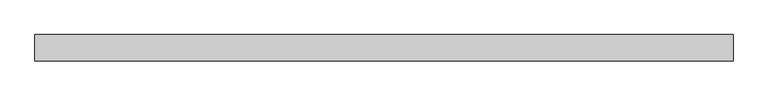
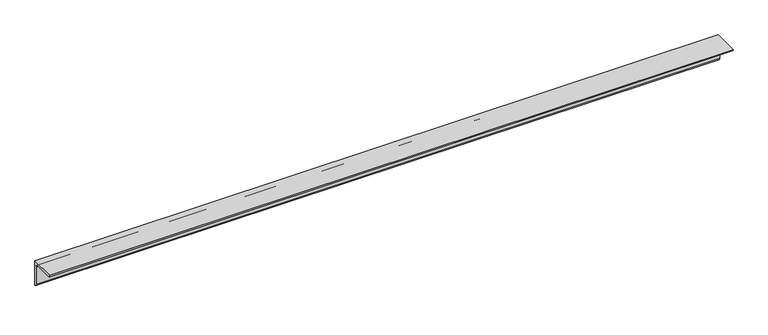
"""IFC4 building model written with IfcOpenShell, lengths in millimetres: member geometry, 0912_Steel Framing_L-KSD3502 : H_SB_AR_S03_L-130x130x12_HBR3."""

from ifc_helpers import new_model, si_unit, point, frame, frame_2d, origin, place, context, project, spatial, polyline, circle_curve, trimmed, segment, composite_curve, outline, extrude, source, transform, mapped, element, save


def member_c4214433(model_context):
    return source(origin(), model_context, "Body", "SweptSolid", [
        extrude(outline(composite_curve([segment(polyline([(36.4, 36.4), (36.4, -93.6)]), True, "CONTINUOUS"), segment(trimmed(circle_curve(frame_2d((36.4, -81.6)), 12.0), [point((36.4, -93.6))], [point((24.4, -81.6))], False, "CARTESIAN"), True, "CONTINUOUS"), segment(polyline([(24.4, -81.6), (24.4, 12.4)]), True, "CONTINUOUS"), segment(trimmed(circle_curve(frame_2d((12.4, 12.4)), 12.0), [point((24.4, 12.4))], [point((12.4, 24.4))], True, "CARTESIAN"), True, "CONTINUOUS"), segment(polyline([(12.4, 24.4), (-81.6, 24.4)]), True, "CONTINUOUS"), segment(trimmed(circle_curve(frame_2d((-81.6, 36.4)), 12.0), [point((-81.6, 24.4))], [point((-93.6, 36.4))], False, "CARTESIAN"), True, "CONTINUOUS"), segment(polyline([(-93.6, 36.4), (36.4, 36.4)]), True, "CONTINUOUS")], self_intersect=False)), frame((-1697.0859301, 0.0, 0.0), z_axis=(1.0, 0.0, 0.0), x_axis=(0.0, 1.0, 0.0)), (0.0, 0.0, 1.0), 3437.7434073),
    ])


if __name__ == "__main__":
    model = new_model("IFC4")
    model_context = context("Model", 3, world=origin())
    ifc_project = project(units=[si_unit("LENGTHUNIT", "METRE", prefix="MILLI")], contexts=[model_context])
    site = spatial("IfcSite", under=ifc_project)
    building = spatial("IfcBuilding", under=site)
    placement = place(None, origin())
    member_shape = member_c4214433(model_context)
    element("IfcMember", 1, ObjectType="0912_Steel Framing_L-KSD3502 : H_SB_AR_S03_L-130x130x12_HBR3", at=placement, inside=building, context=model_context, shape_type="MappedRepresentation", body=[
        mapped(member_shape, transform((0.0, 0.0, 0.0), x_axis=(1.0, 0.0, 0.0), y_axis=(0.0, 1.0, 0.0), z_axis=(0.0, 0.0, 1.0))),
    ])
    save(model, "model.ifc")

# Revit data of these elements
# Type "0912_Steel Framing_L-KSD3502 : H_SB_AR_S03_L-130x130x12_HBR3"
#   k = 25 mm
#   Perimeter = 0.52 m²/m
#   Nominal Weight = 23.40 kgf/m
#   Length [instance default] = 1000 mm
#   b = 130 mm
#   d = 130 mm
#   t = 12 mm
#   x = 36.4 mm
#   y = 36.4 mm
#   A = 2976.00 m²
#   Structural Material [instance default] = Steel, 45-345
# Element 1 (IfcMember, "0912_Steel Framing_L-KSD3502 : H_SB_AR_S03_L-130x130x12_HBR3")
#   Structural Material = Steel ASTM A36
#   Materials on its faces: "Steel ASTM A36"
# Materials
#   "Steel, 45-345": class "Metal", colour RGB 189 187 185, transparency 0, Description = "Steel 345 MPa", Cost = 0
#   "Steel ASTM A36": class "Metal", colour RGB 199 199 199, transparency 0, Description = "Structural steel, ASTM A36 Grade B, mill finish", Cost = 0
